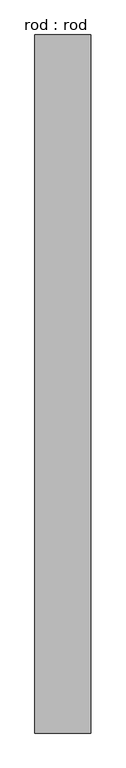
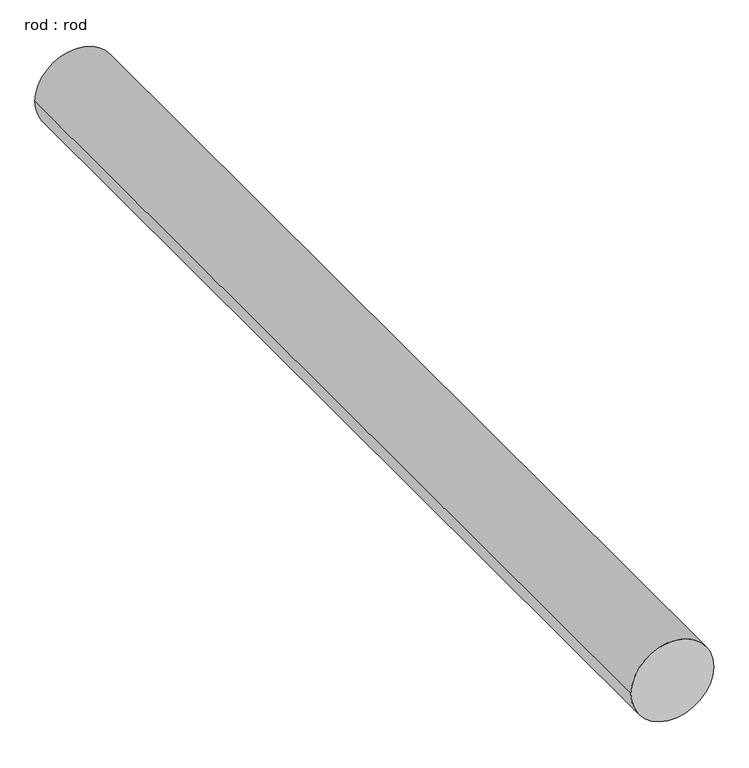
"""IFC4 building model written with IfcOpenShell, lengths in millimetres: proxy geometry, rod : rod."""

import ifcopenshell
import ifcopenshell.guid

model = None  # the IFC model being written
_history = None  # IfcOwnerHistory: only IFC2X3 demands one
_inside = {}  # id of a spatial element -> (the spatial element, [elements in it])
_under = {}  # id of a project, library or spatial element -> (it, [spatial elements below it])
_declared = {}  # id of a project -> (the project, [libraries it declares])
_typed = {}  # id of a type object -> (the type object, [elements of that type])
_made_of = {}  # id of a material, layer set ... -> (it, [elements and type objects made of it])


def new_model(schema):
    """Start an empty IFC model of exactly this schema.

    Asked for "IFC4X3", IfcOpenShell would pick the latest addendum, in which some entities
    have other attributes; the version numbers below select the first issue.
    IFC2X3 requires an IfcOwnerHistory on every rooted entity: one is made here for all.
    """
    global model, _history
    if schema == "IFC4X3":
        model = ifcopenshell.file(schema_version=(4, 3, 0, 0))
    else:
        model = ifcopenshell.file(schema=schema)
    _inside.clear()
    _under.clear()
    _declared.clear()
    _typed.clear()
    _made_of.clear()
    _history = None
    if model.schema == "IFC2X3":
        org = make("IfcOrganization", Name="unknown")
        user = make(
            "IfcPersonAndOrganization",
            ThePerson=make("IfcPerson", FamilyName="unknown"),
            TheOrganization=org,
        )
        app = make(
            "IfcApplication",
            ApplicationDeveloper=org,
            Version="unknown",
            ApplicationFullName="unknown",
            ApplicationIdentifier="unknown",
        )
        _history = make(
            "IfcOwnerHistory",
            OwningUser=user,
            OwningApplication=app,
            ChangeAction="ADDED",
            CreationDate=0,
        )
    return model


def make(cls, **values):
    """One entity of the class cls with the attributes given. An attribute that is None is left unset."""
    return model.create_entity(
        cls, **{name: value for name, value in values.items() if value is not None}
    )


def rooted(cls, **values):
    """An entity with a GlobalId (a new one), such as an element, a storey or a relation."""
    return make(cls, GlobalId=ifcopenshell.guid.new(), OwnerHistory=_history, **values)


def si_unit(unit_type, name, prefix=None):
    """IfcSIUnit, for example si_unit("LENGTHUNIT", "METRE", prefix="MILLI")."""
    return make("IfcSIUnit", UnitType=unit_type, Prefix=prefix, Name=name)


def assignment(units):
    """IfcUnitAssignment: the units of a project."""
    return None if units is None else make("IfcUnitAssignment", Units=units)


def point(xyz):
    """IfcCartesianPoint."""
    return None if xyz is None else make("IfcCartesianPoint", Coordinates=xyz)


def direction(xyz):
    """IfcDirection."""
    return None if xyz is None else make("IfcDirection", DirectionRatios=xyz)


def frame(location, z_axis=None, x_axis=None):
    """IfcAxis2Placement3D, a coordinate frame: its origin and axes. An axis left out is left unset."""
    return make(
        "IfcAxis2Placement3D",
        Location=point(location),
        Axis=direction(z_axis),
        RefDirection=direction(x_axis),
    )


def frame_2d(location, x_axis=None):
    """IfcAxis2Placement2D, a coordinate frame in the plane: its origin and x axis."""
    return make(
        "IfcAxis2Placement2D", Location=point(location), RefDirection=direction(x_axis)
    )


def origin():
    """The frame at (0, 0, 0) with its axes left unset."""
    return frame((0.0, 0.0, 0.0))


def place(relative_to, where):
    """IfcLocalPlacement: puts the frame where relative to a parent placement (None: the world)."""
    return make(
        "IfcLocalPlacement", PlacementRelTo=relative_to, RelativePlacement=where
    )


def context(
    kind, dimensions, precision=None, world=None, true_north=None, identifier=None
):
    """IfcGeometricRepresentationContext, for example the 3D "Model" context."""
    return make(
        "IfcGeometricRepresentationContext",
        ContextIdentifier=identifier,
        ContextType=kind,
        CoordinateSpaceDimension=dimensions,
        Precision=precision,
        WorldCoordinateSystem=world,
        TrueNorth=true_north,
    )


def project(units=None, contexts=None):
    """IfcProject with its units and contexts."""
    return rooted(
        "IfcProject",
        Name="project",
        RepresentationContexts=contexts,
        UnitsInContext=assignment(units),
    )


def spatial(cls, under=None, at=None, **own):
    """A site, building, storey or space (cls), placed at a placement, below another one or the project."""
    s = rooted(cls, ObjectPlacement=at, **own)
    if under is not None:
        _under.setdefault(under.id(), (under, []))[1].append(s)
    return s


def circle_curve(where, radius):
    """IfcCircle in the frame where."""
    return make("IfcCircle", Position=where, Radius=radius)


def trimmed(basis, trim1, trim2, sense, master):
    """IfcTrimmedCurve: the piece of a basis curve between two trims."""
    return make(
        "IfcTrimmedCurve",
        BasisCurve=basis,
        Trim1=trim1,
        Trim2=trim2,
        SenseAgreement=sense,
        MasterRepresentation=master,
    )


def segment(curve, same_sense, transition):
    """IfcCompositeCurveSegment."""
    return make(
        "IfcCompositeCurveSegment",
        Transition=transition,
        SameSense=same_sense,
        ParentCurve=curve,
    )


def composite_curve(segments, self_intersect=None):
    """IfcCompositeCurve: segments joined end to end."""
    return make("IfcCompositeCurve", Segments=segments, SelfIntersect=self_intersect)


def outline(outer, holes=None, kind="AREA"):
    """IfcArbitraryClosedProfileDef: a profile drawn as a closed curve; with holes, ...WithVoids."""
    if holes is None:
        return make("IfcArbitraryClosedProfileDef", ProfileType=kind, OuterCurve=outer)
    return make(
        "IfcArbitraryProfileDefWithVoids",
        ProfileType=kind,
        OuterCurve=outer,
        InnerCurves=holes,
    )


def extrude(swept, where, along, depth):
    """IfcExtrudedAreaSolid: the profile swept, set in the frame where, extruded along a direction by depth."""
    return make(
        "IfcExtrudedAreaSolid",
        SweptArea=swept,
        Position=where,
        ExtrudedDirection=direction(along),
        Depth=depth,
    )


def shape(context_of_items, identifier, shape_type, items):
    """IfcShapeRepresentation: the items that make up one representation, for example the "Body"."""
    return make(
        "IfcShapeRepresentation",
        ContextOfItems=context_of_items,
        RepresentationIdentifier=identifier,
        RepresentationType=shape_type,
        Items=items,
    )


def source(mapping_origin, context_of_items, identifier, shape_type, items):
    """IfcRepresentationMap: a shape defined once, which mapped items show again and again."""
    return make(
        "IfcRepresentationMap",
        MappingOrigin=mapping_origin,
        MappedRepresentation=shape(context_of_items, identifier, shape_type, items),
    )


def transform(
    local_origin,
    x_axis=None,
    y_axis=None,
    z_axis=None,
    scale=None,
    scale2=None,
    scale3=None,
    uniform=True,
):
    """IfcCartesianTransformationOperator3D, or its non-uniform kind. x_axis, y_axis, z_axis: its Axis1, 2, 3."""
    if uniform:
        return make(
            "IfcCartesianTransformationOperator3D",
            Axis1=direction(x_axis),
            Axis2=direction(y_axis),
            LocalOrigin=point(local_origin),
            Scale=scale,
            Axis3=direction(z_axis),
        )
    return make(
        "IfcCartesianTransformationOperator3DnonUniform",
        Axis1=direction(x_axis),
        Axis2=direction(y_axis),
        LocalOrigin=point(local_origin),
        Scale=scale,
        Axis3=direction(z_axis),
        Scale2=scale2,
        Scale3=scale3,
    )


def mapped(mapping_source, mapping_target):
    """IfcMappedItem: shows the shape of a source again, moved by a transform."""
    return make(
        "IfcMappedItem", MappingSource=mapping_source, MappingTarget=mapping_target
    )


def made_of(thing, what):
    """Note that an element or type object is made of a material, layer set ...; save() writes the relation."""
    if what is not None:
        _made_of.setdefault(what.id(), (what, []))[1].append(thing)
    return thing


def element(
    cls,
    number,
    at=None,
    inside=None,
    cuts=None,
    type_object=None,
    material=None,
    context=None,
    identifier="Body",
    shape_type=None,
    held_by="IfcProductDefinitionShape",
    body=None,
    shapes=None,
    **own,
):
    """One element of the class cls, such as IfcWall. Its Tag is "e" and its number.

    at: its placement. inside: the storey or other place that contains it. cuts: it is an
    opening in that element (IfcRelVoidsElement). A single representation is given by context,
    identifier, shape_type and body (its items); several are given by shapes. held_by: the class
    of the entity that holds the representations. save() writes the other relations.
    """
    e = rooted(cls, Tag="e%d" % number, ObjectPlacement=at, **own)
    if body is not None:
        shapes = [shape(context, identifier, shape_type, body)]
    if shapes is not None:
        e.Representation = make(held_by, Representations=shapes)
    if inside is not None:
        _inside.setdefault(inside.id(), (inside, []))[1].append(e)
    if cuts is not None:
        rooted(
            "IfcRelVoidsElement", RelatingBuildingElement=cuts, RelatedOpeningElement=e
        )
    if type_object is not None:
        _typed.setdefault(type_object.id(), (type_object, []))[1].append(e)
    return made_of(e, material)


def aggregate(whole, parts):
    """IfcRelAggregates: a whole, such as a stair, and the parts it consists of."""
    return rooted("IfcRelAggregates", RelatingObject=whole, RelatedObjects=parts)


def save(model, path):
    """Write the relations noted so far, then the file.

    IfcRelAggregates (storeys below a building ...), IfcRelContainedInSpatialStructure (elements
    in a storey), IfcRelDefinesByType, IfcRelAssociatesMaterial and IfcRelDeclares: one each for
    every whole, place, type object, material and project.
    """
    for whole, parts in _under.values():
        aggregate(whole, parts)
    for where, things in _inside.values():
        rooted(
            "IfcRelContainedInSpatialStructure",
            RelatedElements=things,
            RelatingStructure=where,
        )
    for kind, things in _typed.values():
        rooted("IfcRelDefinesByType", RelatedObjects=things, RelatingType=kind)
    for what, things in _made_of.values():
        rooted("IfcRelAssociatesMaterial", RelatedObjects=things, RelatingMaterial=what)
    for by, libraries in _declared.values():
        rooted("IfcRelDeclares", RelatingContext=by, RelatedDefinitions=libraries)
    model.write(path)


def rod_rod_b2d37f7d(model_context):
    return source(origin(), model_context, "Body", "SweptSolid", [
        extrude(outline(composite_curve([segment(trimmed(circle_curve(frame_2d((0.0108462, 0.0)), 200.0), [point((0.0108462, 200.0))], [point((0.0108462, -200.0))], False, "CARTESIAN"), True, "CONTINUOUS"), segment(trimmed(circle_curve(frame_2d((0.0108462, 0.0)), 200.0), [point((0.0108462, -200.0))], [point((0.0108462, 200.0))], False, "CARTESIAN"), True, "CONTINUOUS")], self_intersect=False)), frame((0.0, 1592.7286153, 0.0), z_axis=(0.0, 1.0, 0.0), x_axis=(0.0, 0.0, 1.0)), (0.0, 0.0, 1.0), 5000.0),
    ])


if __name__ == "__main__":
    model = new_model("IFC4")
    model_context = context("Model", 3, world=origin())
    ifc_project = project(units=[si_unit("LENGTHUNIT", "METRE", prefix="MILLI")], contexts=[model_context])
    site = spatial("IfcSite", under=ifc_project)
    building = spatial("IfcBuilding", under=site)
    placement = place(None, origin())
    rod_rod_shape = rod_rod_b2d37f7d(model_context)
    element("IfcBuildingElementProxy", 1, Name="rod : rod", ObjectType="rod : rod", at=placement, inside=building, context=model_context, shape_type="MappedRepresentation", body=[
        mapped(rod_rod_shape, transform((0.0, 0.0, 0.0), x_axis=(1.0, 0.0, 0.0), y_axis=(0.0, 1.0, 0.0), z_axis=(0.0, 0.0, 1.0))),
    ])
    save(model, "model.ifc")

# Revit data of these elements
# Type "rod : rod"
#   Default Elevation = 0
